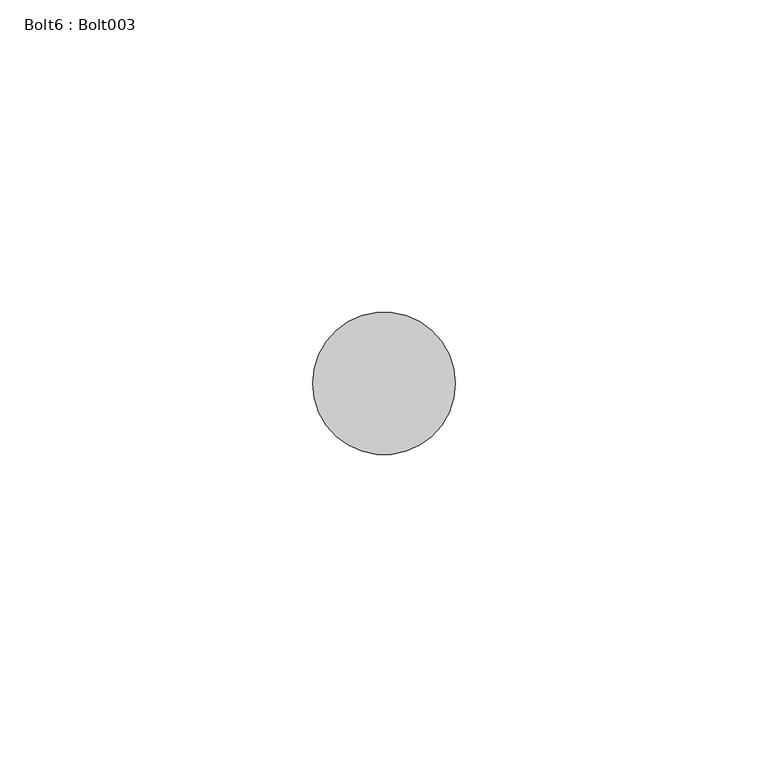
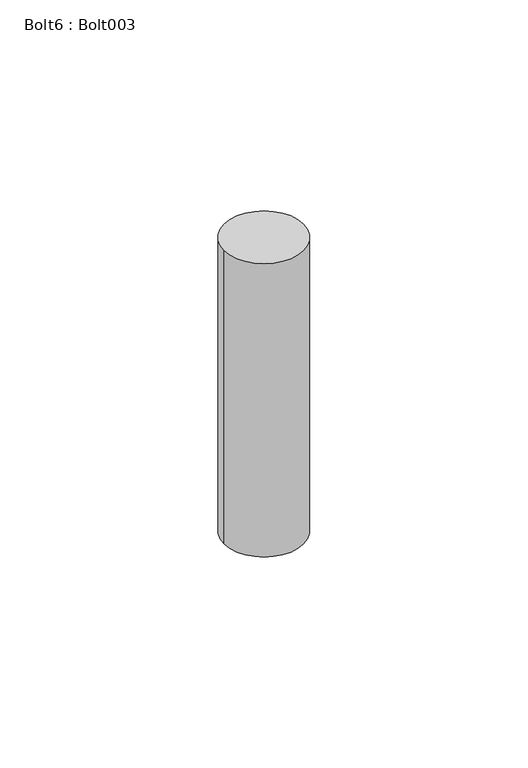
"""IFC4 building model written with IfcOpenShell, lengths in millimetres: proxy geometry, Bolt6 : Bolt003."""

import ifcopenshell
import ifcopenshell.guid

model = None  # the IFC model being written
_history = None  # IfcOwnerHistory: only IFC2X3 demands one
_inside = {}  # id of a spatial element -> (the spatial element, [elements in it])
_under = {}  # id of a project, library or spatial element -> (it, [spatial elements below it])
_declared = {}  # id of a project -> (the project, [libraries it declares])
_typed = {}  # id of a type object -> (the type object, [elements of that type])
_made_of = {}  # id of a material, layer set ... -> (it, [elements and type objects made of it])


def new_model(schema):
    """Start an empty IFC model of exactly this schema.

    Asked for "IFC4X3", IfcOpenShell would pick the latest addendum, in which some entities
    have other attributes; the version numbers below select the first issue.
    IFC2X3 requires an IfcOwnerHistory on every rooted entity: one is made here for all.
    """
    global model, _history
    if schema == "IFC4X3":
        model = ifcopenshell.file(schema_version=(4, 3, 0, 0))
    else:
        model = ifcopenshell.file(schema=schema)
    _inside.clear()
    _under.clear()
    _declared.clear()
    _typed.clear()
    _made_of.clear()
    _history = None
    if model.schema == "IFC2X3":
        org = make("IfcOrganization", Name="unknown")
        user = make(
            "IfcPersonAndOrganization",
            ThePerson=make("IfcPerson", FamilyName="unknown"),
            TheOrganization=org,
        )
        app = make(
            "IfcApplication",
            ApplicationDeveloper=org,
            Version="unknown",
            ApplicationFullName="unknown",
            ApplicationIdentifier="unknown",
        )
        _history = make(
            "IfcOwnerHistory",
            OwningUser=user,
            OwningApplication=app,
            ChangeAction="ADDED",
            CreationDate=0,
        )
    return model


def make(cls, **values):
    """One entity of the class cls with the attributes given. An attribute that is None is left unset."""
    return model.create_entity(
        cls, **{name: value for name, value in values.items() if value is not None}
    )


def rooted(cls, **values):
    """An entity with a GlobalId (a new one), such as an element, a storey or a relation."""
    return make(cls, GlobalId=ifcopenshell.guid.new(), OwnerHistory=_history, **values)


def si_unit(unit_type, name, prefix=None):
    """IfcSIUnit, for example si_unit("LENGTHUNIT", "METRE", prefix="MILLI")."""
    return make("IfcSIUnit", UnitType=unit_type, Prefix=prefix, Name=name)


def assignment(units):
    """IfcUnitAssignment: the units of a project."""
    return None if units is None else make("IfcUnitAssignment", Units=units)


def point(xyz):
    """IfcCartesianPoint."""
    return None if xyz is None else make("IfcCartesianPoint", Coordinates=xyz)


def direction(xyz):
    """IfcDirection."""
    return None if xyz is None else make("IfcDirection", DirectionRatios=xyz)


def frame(location, z_axis=None, x_axis=None):
    """IfcAxis2Placement3D, a coordinate frame: its origin and axes. An axis left out is left unset."""
    return make(
        "IfcAxis2Placement3D",
        Location=point(location),
        Axis=direction(z_axis),
        RefDirection=direction(x_axis),
    )


def frame_2d(location, x_axis=None):
    """IfcAxis2Placement2D, a coordinate frame in the plane: its origin and x axis."""
    return make(
        "IfcAxis2Placement2D", Location=point(location), RefDirection=direction(x_axis)
    )


def origin():
    """The frame at (0, 0, 0) with its axes left unset."""
    return frame((0.0, 0.0, 0.0))


def place(relative_to, where):
    """IfcLocalPlacement: puts the frame where relative to a parent placement (None: the world)."""
    return make(
        "IfcLocalPlacement", PlacementRelTo=relative_to, RelativePlacement=where
    )


def context(
    kind, dimensions, precision=None, world=None, true_north=None, identifier=None
):
    """IfcGeometricRepresentationContext, for example the 3D "Model" context."""
    return make(
        "IfcGeometricRepresentationContext",
        ContextIdentifier=identifier,
        ContextType=kind,
        CoordinateSpaceDimension=dimensions,
        Precision=precision,
        WorldCoordinateSystem=world,
        TrueNorth=true_north,
    )


def project(units=None, contexts=None):
    """IfcProject with its units and contexts."""
    return rooted(
        "IfcProject",
        Name="project",
        RepresentationContexts=contexts,
        UnitsInContext=assignment(units),
    )


def spatial(cls, under=None, at=None, **own):
    """A site, building, storey or space (cls), placed at a placement, below another one or the project."""
    s = rooted(cls, ObjectPlacement=at, **own)
    if under is not None:
        _under.setdefault(under.id(), (under, []))[1].append(s)
    return s


def circle_curve(where, radius):
    """IfcCircle in the frame where."""
    return make("IfcCircle", Position=where, Radius=radius)


def trimmed(basis, trim1, trim2, sense, master):
    """IfcTrimmedCurve: the piece of a basis curve between two trims."""
    return make(
        "IfcTrimmedCurve",
        BasisCurve=basis,
        Trim1=trim1,
        Trim2=trim2,
        SenseAgreement=sense,
        MasterRepresentation=master,
    )


def segment(curve, same_sense, transition):
    """IfcCompositeCurveSegment."""
    return make(
        "IfcCompositeCurveSegment",
        Transition=transition,
        SameSense=same_sense,
        ParentCurve=curve,
    )


def composite_curve(segments, self_intersect=None):
    """IfcCompositeCurve: segments joined end to end."""
    return make("IfcCompositeCurve", Segments=segments, SelfIntersect=self_intersect)


def outline(outer, holes=None, kind="AREA"):
    """IfcArbitraryClosedProfileDef: a profile drawn as a closed curve; with holes, ...WithVoids."""
    if holes is None:
        return make("IfcArbitraryClosedProfileDef", ProfileType=kind, OuterCurve=outer)
    return make(
        "IfcArbitraryProfileDefWithVoids",
        ProfileType=kind,
        OuterCurve=outer,
        InnerCurves=holes,
    )


def extrude(swept, where, along, depth):
    """IfcExtrudedAreaSolid: the profile swept, set in the frame where, extruded along a direction by depth."""
    return make(
        "IfcExtrudedAreaSolid",
        SweptArea=swept,
        Position=where,
        ExtrudedDirection=direction(along),
        Depth=depth,
    )


def shape(context_of_items, identifier, shape_type, items):
    """IfcShapeRepresentation: the items that make up one representation, for example the "Body"."""
    return make(
        "IfcShapeRepresentation",
        ContextOfItems=context_of_items,
        RepresentationIdentifier=identifier,
        RepresentationType=shape_type,
        Items=items,
    )


def source(mapping_origin, context_of_items, identifier, shape_type, items):
    """IfcRepresentationMap: a shape defined once, which mapped items show again and again."""
    return make(
        "IfcRepresentationMap",
        MappingOrigin=mapping_origin,
        MappedRepresentation=shape(context_of_items, identifier, shape_type, items),
    )


def transform(
    local_origin,
    x_axis=None,
    y_axis=None,
    z_axis=None,
    scale=None,
    scale2=None,
    scale3=None,
    uniform=True,
):
    """IfcCartesianTransformationOperator3D, or its non-uniform kind. x_axis, y_axis, z_axis: its Axis1, 2, 3."""
    if uniform:
        return make(
            "IfcCartesianTransformationOperator3D",
            Axis1=direction(x_axis),
            Axis2=direction(y_axis),
            LocalOrigin=point(local_origin),
            Scale=scale,
            Axis3=direction(z_axis),
        )
    return make(
        "IfcCartesianTransformationOperator3DnonUniform",
        Axis1=direction(x_axis),
        Axis2=direction(y_axis),
        LocalOrigin=point(local_origin),
        Scale=scale,
        Axis3=direction(z_axis),
        Scale2=scale2,
        Scale3=scale3,
    )


def mapped(mapping_source, mapping_target):
    """IfcMappedItem: shows the shape of a source again, moved by a transform."""
    return make(
        "IfcMappedItem", MappingSource=mapping_source, MappingTarget=mapping_target
    )


def made_of(thing, what):
    """Note that an element or type object is made of a material, layer set ...; save() writes the relation."""
    if what is not None:
        _made_of.setdefault(what.id(), (what, []))[1].append(thing)
    return thing


def element(
    cls,
    number,
    at=None,
    inside=None,
    cuts=None,
    type_object=None,
    material=None,
    context=None,
    identifier="Body",
    shape_type=None,
    held_by="IfcProductDefinitionShape",
    body=None,
    shapes=None,
    **own,
):
    """One element of the class cls, such as IfcWall. Its Tag is "e" and its number.

    at: its placement. inside: the storey or other place that contains it. cuts: it is an
    opening in that element (IfcRelVoidsElement). A single representation is given by context,
    identifier, shape_type and body (its items); several are given by shapes. held_by: the class
    of the entity that holds the representations. save() writes the other relations.
    """
    e = rooted(cls, Tag="e%d" % number, ObjectPlacement=at, **own)
    if body is not None:
        shapes = [shape(context, identifier, shape_type, body)]
    if shapes is not None:
        e.Representation = make(held_by, Representations=shapes)
    if inside is not None:
        _inside.setdefault(inside.id(), (inside, []))[1].append(e)
    if cuts is not None:
        rooted(
            "IfcRelVoidsElement", RelatingBuildingElement=cuts, RelatedOpeningElement=e
        )
    if type_object is not None:
        _typed.setdefault(type_object.id(), (type_object, []))[1].append(e)
    return made_of(e, material)


def aggregate(whole, parts):
    """IfcRelAggregates: a whole, such as a stair, and the parts it consists of."""
    return rooted("IfcRelAggregates", RelatingObject=whole, RelatedObjects=parts)


def save(model, path):
    """Write the relations noted so far, then the file.

    IfcRelAggregates (storeys below a building ...), IfcRelContainedInSpatialStructure (elements
    in a storey), IfcRelDefinesByType, IfcRelAssociatesMaterial and IfcRelDeclares: one each for
    every whole, place, type object, material and project.
    """
    for whole, parts in _under.values():
        aggregate(whole, parts)
    for where, things in _inside.values():
        rooted(
            "IfcRelContainedInSpatialStructure",
            RelatedElements=things,
            RelatingStructure=where,
        )
    for kind, things in _typed.values():
        rooted("IfcRelDefinesByType", RelatedObjects=things, RelatingType=kind)
    for what, things in _made_of.values():
        rooted("IfcRelAssociatesMaterial", RelatedObjects=things, RelatingMaterial=what)
    for by, libraries in _declared.values():
        rooted("IfcRelDeclares", RelatingContext=by, RelatedDefinitions=libraries)
    model.write(path)


def bolt6_bolt003_a672977d(model_context):
    return source(origin(), model_context, "Body", "SweptSolid", [
        extrude(outline(composite_curve([segment(trimmed(circle_curve(frame_2d((5172.3828124, 1896.5882072)), 11.4045168), [point((5160.9782956, 1896.5882072))], [point((5183.7873292, 1896.5882072))], False, "CARTESIAN"), True, "CONTINUOUS"), segment(trimmed(circle_curve(frame_2d((5172.3828124, 1896.5882072)), 11.4045168), [point((5183.7873292, 1896.5882072))], [point((5160.9782956, 1896.5882072))], False, "CARTESIAN"), True, "CONTINUOUS")], self_intersect=False)), frame((0.0, 0.0, 36645.5959962), z_axis=(0.0, 0.0, 1.0), x_axis=(1.0, 0.0, 0.0)), (0.0, 0.0, 1.0), 88.9),
    ])


if __name__ == "__main__":
    model = new_model("IFC4")
    model_context = context("Model", 3, world=origin())
    ifc_project = project(units=[si_unit("LENGTHUNIT", "METRE", prefix="MILLI")], contexts=[model_context])
    site = spatial("IfcSite", under=ifc_project)
    building = spatial("IfcBuilding", under=site)
    placement = place(None, origin())
    bolt6_bolt003_shape = bolt6_bolt003_a672977d(model_context)
    element("IfcBuildingElementProxy", 1, Name="Bolt6 : Bolt003", ObjectType="Bolt6 : Bolt003", at=placement, inside=building, context=model_context, shape_type="MappedRepresentation", body=[
        mapped(bolt6_bolt003_shape, transform((0.0, 0.0, 0.0), x_axis=(1.0, 0.0, 0.0), y_axis=(0.0, 1.0, 0.0), z_axis=(0.0, 0.0, 1.0))),
    ])
    save(model, "model.ifc")

# Revit data of these elements
# Type "Bolt6 : Bolt003"
#   NameOverride = "Bolt003"
# Element 1 (IfcBuildingElementProxy, "Bolt6 : Bolt003")
#   Materials on its faces: "TUBE STEEL STRINGER WELDED TO ANCHORED STEEL PLATE - SEE STRUCT DWGS"
# Materials
#   "TUBE STEEL STRINGER WELDED TO ANCHORED STEEL PLATE - SEE STRUCT DWGS": class "Unassigned", colour RGB 128 128 128, transparency 0, Cost = 0
